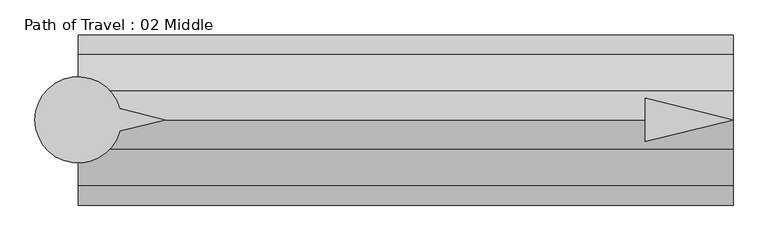
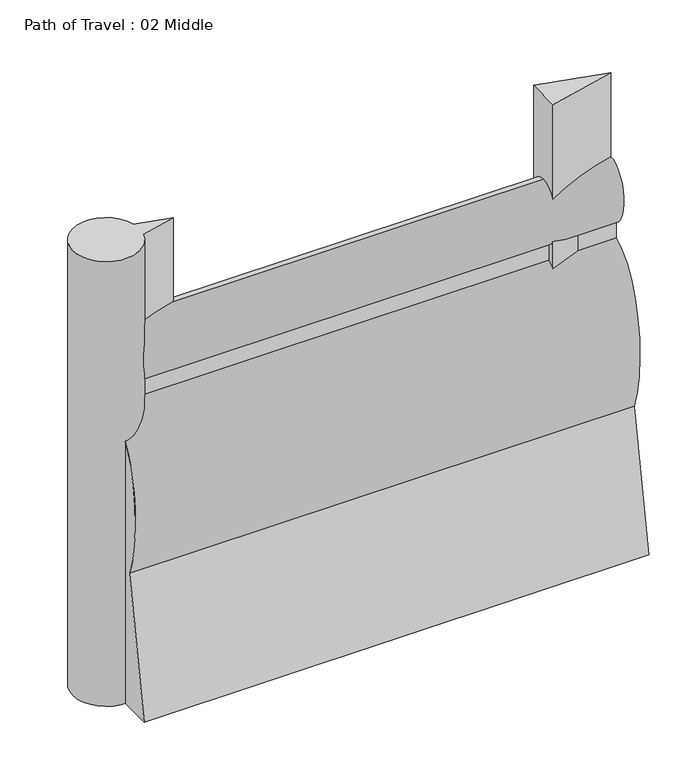
"""IFC4 building model written with IfcOpenShell, lengths in millimetres: proxy geometry, Path of Travel : 02 Middle."""

from ifc_helpers import new_model, si_unit, point, frame, frame_2d, origin, origin_with_axes, place, context, project, spatial, polyline, circle_curve, ellipse_curve, trimmed, segment, composite_curve, outline, extrude, source, transform, mapped, element, save
from ifc_brep_helpers import plane_surface, extruded_surface, advanced_brep


def path_of_travel_02_middle_d2f13536(model_context):
    return source(origin(), model_context, "Body", "SolidModel", [
        advanced_brep(
        [(227.5554837, 0.0, 1727.2), (227.5554837, 42.9018657, 1436.6534209), (227.5554837, 42.9018657, 1363.4763406), (227.5554837, 184.1186263, 643.4144547), (227.5554837, 297.5699544, 0.0), (227.5554837, 145.6574193, 0.0), (227.5554837, 0.0, 584.2), (227.5554837, -145.6574193, 0.0), (227.5554837, -297.5699544, 0.0), (227.5554837, -184.1186263, 643.4144547), (227.5554837, -42.9018657, 1363.4763406), (227.5554837, -42.9018657, 1436.6534209), (2513.5554837, 0.0, 1727.2), (2513.5554837, -42.9018657, 1436.6534209), (2513.5554837, -42.9018657, 1363.4763406), (2513.5554837, -184.1186263, 643.4144547), (2513.5554837, -297.5699544, 0.0), (2513.5554837, -145.6574193, 0.0), (2513.5554837, 0.0, 584.2), (2513.5554837, 145.6574193, 0.0), (2513.5554837, 297.5699544, 0.0), (2513.5554837, 184.1186263, 643.4144547), (2513.5554837, 42.9018657, 1363.4763406), (2513.5554837, 42.9018657, 1436.6534209)],
        [
            (0, 1, ellipse_curve(frame((227.5554837, 0.0, 1574.8), z_axis=(-1.0, 0.0, 0.0), x_axis=(0.0, 0.0, 1.0)), 152.4, 101.6)),
            (1, 2),
            (2, 3, ellipse_curve(frame((227.5554837, 0.0, 914.4), z_axis=(-1.0, 0.0, 0.0), x_axis=(0.0, 0.0, -1.0)), 457.2, 228.6)),
            (3, 4),
            (4, 5),
            (5, 6),
            (6, 7),
            (7, 8),
            (8, 9),
            (9, 10, ellipse_curve(frame((227.5554837, 0.0, 914.4), z_axis=(-1.0, 0.0, 0.0), x_axis=(0.0, 0.0, -1.0)), 457.2, 228.6)),
            (10, 11),
            (11, 0, ellipse_curve(frame((227.5554837, 0.0, 1574.8), z_axis=(-1.0, 0.0, 0.0), x_axis=(0.0, 0.0, 1.0)), 152.4, 101.6)),
            (12, 13, ellipse_curve(frame((2513.5554837, 0.0, 1574.8), z_axis=(1.0, 0.0, 0.0), x_axis=(0.0, 0.0, 1.0)), 152.4, 101.6)),
            (13, 14),
            (14, 15, ellipse_curve(frame((2513.5554837, 0.0, 914.4), z_axis=(1.0, 0.0, 0.0), x_axis=(0.0, 0.0, -1.0)), 457.2, 228.6)),
            (15, 16),
            (16, 17),
            (17, 18),
            (18, 19),
            (19, 20),
            (20, 21),
            (21, 22, ellipse_curve(frame((2513.5554837, 0.0, 914.4), z_axis=(1.0, 0.0, 0.0), x_axis=(0.0, 0.0, -1.0)), 457.2, 228.6)),
            (22, 23),
            (23, 12, ellipse_curve(frame((2513.5554837, 0.0, 1574.8), z_axis=(1.0, 0.0, 0.0), x_axis=(0.0, 0.0, 1.0)), 152.4, 101.6)),
            (0, 12),
            (23, 1),
            (22, 2),
            (21, 3),
            (20, 4),
            (19, 5),
            (18, 6),
            (17, 7),
            (16, 8),
            (15, 9),
            (14, 10),
            (13, 11),
        ],
        [
            plane_surface(frame((227.5554837, 0.0, 0.0), z_axis=(-1.0, 0.0, 0.0), x_axis=(0.0, 0.0, 1.0))),
            plane_surface(frame((2513.5554837, 0.0, 0.0), z_axis=(1.0, 0.0, 0.0), x_axis=(0.0, 0.0, 1.0))),
            extruded_surface(trimmed(ellipse_curve(frame((2513.5554837, 0.0, 1574.8), z_axis=(-1.0, 0.0, 0.0), x_axis=(0.0, 0.0, 1.0)), 152.4, 101.6), [point((2513.5554837, 0.0, 1727.2))], [point((2513.5554837, 42.9018657, 1436.6534209))], True, "CARTESIAN"), (-2286.0, 0.0, 0.0), 2286.0),
            plane_surface(frame((227.5554837, 42.9018657, 1436.6534209), z_axis=(0.0, 1.0, 0.0), x_axis=(1.0, 0.0, 0.0))),
            extruded_surface(trimmed(ellipse_curve(frame((2513.5554837, 0.0, 914.4), z_axis=(-1.0, 0.0, 0.0), x_axis=(0.0, 0.0, -1.0)), 457.2, 228.6), [point((2513.5554837, 42.9018657, 1363.4763406))], [point((2513.5554837, 184.1186263, 643.4144547))], True, "CARTESIAN"), (-2286.0, 0.0, 0.0), 2286.0),
            plane_surface(frame((227.5554837, 184.1186263, 643.4144547), z_axis=(0.0, 0.9848077530122078, 0.1736481776669322), x_axis=(1.0, 0.0, 0.0))),
            plane_surface(frame((227.5554837, 297.5699544, 0.0), z_axis=(0.0, 0.0, -1.0), x_axis=(1.0, 0.0, 0.0))),
            plane_surface(frame((227.5554837, 145.6574193, 0.0), z_axis=(0.0, -0.9702957262760199, -0.2419218955995739), x_axis=(1.0, 0.0, 0.0))),
            plane_surface(frame((227.5554837, 0.0, 584.2), z_axis=(0.0, 0.9702957262759961, -0.24192189559966923), x_axis=(1.0, 0.0, 0.0))),
            plane_surface(frame((227.5554837, -145.6574193, 0.0), z_axis=(0.0, 0.0, -1.0), x_axis=(1.0, 0.0, 0.0))),
            plane_surface(frame((227.5554837, -297.5699544, 0.0), z_axis=(0.0, -0.984807753012208, 0.17364817766693066), x_axis=(1.0, 0.0, 0.0))),
            extruded_surface(trimmed(ellipse_curve(frame((2513.5554837, 0.0, 914.4), z_axis=(-1.0, 0.0, 0.0), x_axis=(0.0, 0.0, -1.0)), 457.2, 228.6), [point((2513.5554837, -184.1186263, 643.4144547))], [point((2513.5554837, -42.9018657, 1363.4763406))], True, "CARTESIAN"), (-2286.0, 0.0, 0.0), 2286.0),
            plane_surface(frame((227.5554837, -42.9018657, 1363.4763406), z_axis=(0.0, -1.0, 0.0), x_axis=(1.0, 0.0, 0.0))),
            extruded_surface(trimmed(ellipse_curve(frame((2513.5554837, 0.0, 1574.8), z_axis=(-1.0, 0.0, 0.0), x_axis=(0.0, 0.0, 1.0)), 152.4, 101.6), [point((2513.5554837, -42.9018657, 1436.6534209))], [point((2513.5554837, 0.0, 1727.2))], True, "CARTESIAN"), (-2286.0, 0.0, 0.0), 2286.0),
        ],
        [
            (0, [[1, 2, 3, 4, 5, 6, 7, 8, 9, 10, 11, 12]]),
            (1, [[13, 14, 15, 16, 17, 18, 19, 20, 21, 22, 23, 24]]),
            (2, [[-1, 25, -24, 26]]),
            (3, [[-2, -26, -23, 27]]),
            (4, [[-3, -27, -22, 28]]),
            (5, [[-4, -28, -21, 29]]),
            (6, [[-5, -29, -20, 30]]),
            (7, [[-6, -30, -19, 31]]),
            (8, [[-7, -31, -18, 32]]),
            (9, [[-8, -32, -17, 33]]),
            (10, [[-9, -33, -16, 34]]),
            (11, [[-10, -34, -15, 35]]),
            (12, [[-11, -35, -14, 36]]),
            (13, [[-12, -36, -13, -25]]),
        ],
    ),
        extrude(outline(polyline([(2207.5503371, 76.2006338), (2513.5554837, 0.0), (2207.5503371, -76.2006338), (2207.5503371, 76.2006338)])), origin_with_axes(), (0.0, 0.0, 1.0), 2129.5973753),
        extrude(outline(composite_curve([segment(polyline([(372.7837828, 39.4440225), (531.182385, 0.0), (372.7837828, -39.4440225)]), True, "CONTINUOUS"), segment(trimmed(circle_curve(frame_2d((227.2200886, 0.0)), 150.8131956), [point((372.7837828, -39.4440225))], [point((372.7837828, 39.4440225))], False, "CARTESIAN"), True, "CONTINUOUS")], self_intersect=False)), origin_with_axes(), (0.0, 0.0, 1.0), 2129.5973753),
    ])


if __name__ == "__main__":
    model = new_model("IFC4")
    model_context = context("Model", 3, world=origin())
    ifc_project = project(units=[si_unit("LENGTHUNIT", "METRE", prefix="MILLI")], contexts=[model_context])
    site = spatial("IfcSite", under=ifc_project)
    building = spatial("IfcBuilding", under=site)
    placement = place(None, origin())
    path_of_travel_02_middle_shape = path_of_travel_02_middle_d2f13536(model_context)
    element("IfcBuildingElementProxy", 1, Name="Path of Travel : 02 Middle", ObjectType="Path of Travel : 02 Middle", at=placement, inside=building, context=model_context, shape_type="MappedRepresentation", body=[
        mapped(path_of_travel_02_middle_shape, transform((0.0, 0.0, 0.0), x_axis=(1.0, 0.0, 0.0), y_axis=(0.0, 1.0, 0.0), z_axis=(0.0, 0.0, 1.0))),
    ])
    save(model, "model.ifc")

# Revit data of these elements
# Type "Path of Travel : 02 Middle"
#   Path of Egress [instance default] = 4' - 0"
#   built-in parameter 1001306 [instance default] = 4 (stored number, unit not read)
#   Dot at Start = no
#   Arrow in Middle = yes
#   Arrow at End = no
#   Egress Path = none
# Element 1 (IfcBuildingElementProxy, "Path of Travel : 02 Middle")
#   Path of Egress = 7' - 6"
#   built-in parameter 1001306 = 7.5 (stored number, unit not read)
#   Materials on its faces: "Egress Path Solid", "solid"
# Materials
#   "Egress Path Solid": class "Unassigned", colour RGB 255 128 64, transparency 0.75, Comments = "Rendering appearance not upgraded "
#   "solid": class "Generic", colour RGB 120 120 120, transparency 0, Cost = 0
